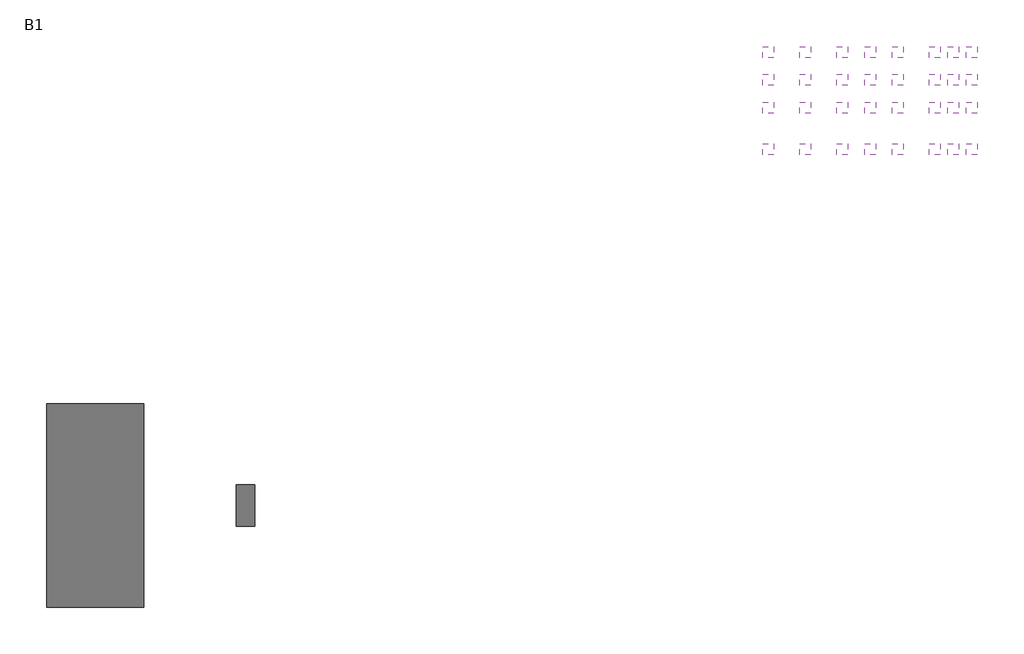
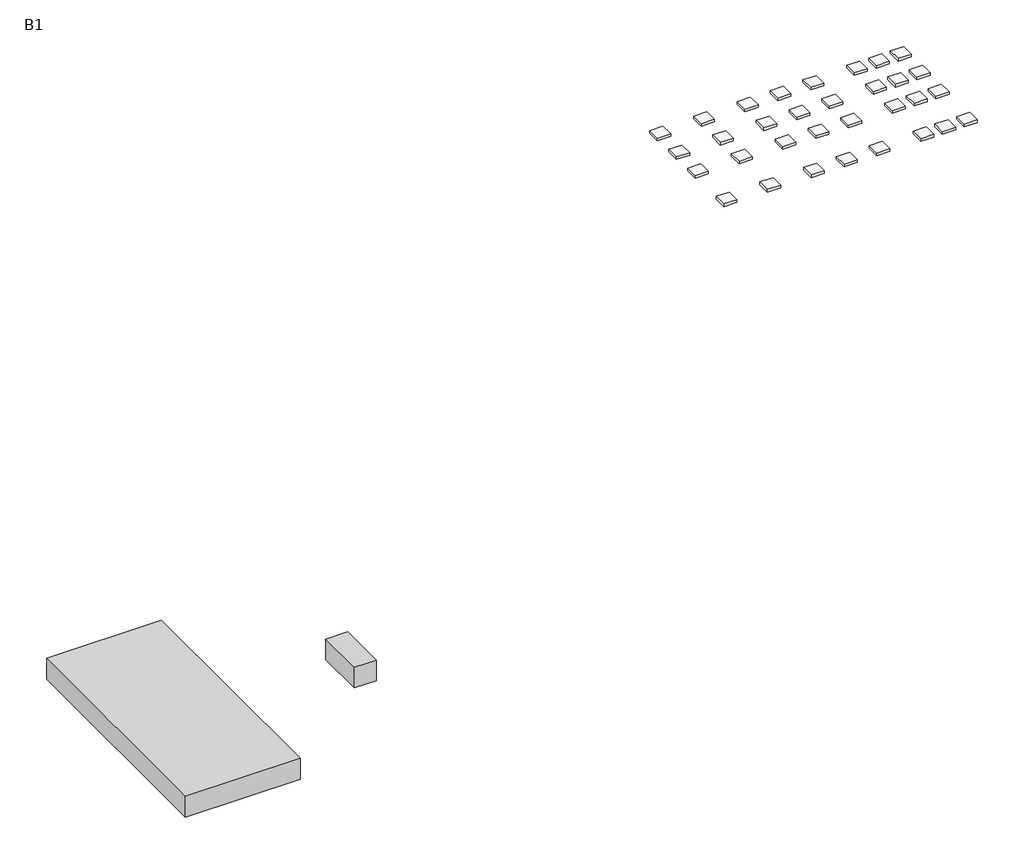
# One storey: 32 slabs, 2 proxies.
"""IFC4 building model written with IfcOpenShell, lengths in millimetres."""

import ifcopenshell
import ifcopenshell.guid

model = None  # the IFC model being written
_history = None  # IfcOwnerHistory: only IFC2X3 demands one
_inside = {}  # id of a spatial element -> (the spatial element, [elements in it])
_under = {}  # id of a project, library or spatial element -> (it, [spatial elements below it])
_declared = {}  # id of a project -> (the project, [libraries it declares])
_typed = {}  # id of a type object -> (the type object, [elements of that type])
_made_of = {}  # id of a material, layer set ... -> (it, [elements and type objects made of it])


def new_model(schema):
    """Start an empty IFC model of exactly this schema.

    Asked for "IFC4X3", IfcOpenShell would pick the latest addendum, in which some entities
    have other attributes; the version numbers below select the first issue.
    IFC2X3 requires an IfcOwnerHistory on every rooted entity: one is made here for all.
    """
    global model, _history
    if schema == "IFC4X3":
        model = ifcopenshell.file(schema_version=(4, 3, 0, 0))
    else:
        model = ifcopenshell.file(schema=schema)
    _inside.clear()
    _under.clear()
    _declared.clear()
    _typed.clear()
    _made_of.clear()
    _history = None
    if model.schema == "IFC2X3":
        org = make("IfcOrganization", Name="unknown")
        user = make(
            "IfcPersonAndOrganization",
            ThePerson=make("IfcPerson", FamilyName="unknown"),
            TheOrganization=org,
        )
        app = make(
            "IfcApplication",
            ApplicationDeveloper=org,
            Version="unknown",
            ApplicationFullName="unknown",
            ApplicationIdentifier="unknown",
        )
        _history = make(
            "IfcOwnerHistory",
            OwningUser=user,
            OwningApplication=app,
            ChangeAction="ADDED",
            CreationDate=0,
        )
    return model


def make(cls, **values):
    """One entity of the class cls with the attributes given. An attribute that is None is left unset."""
    return model.create_entity(
        cls, **{name: value for name, value in values.items() if value is not None}
    )


def rooted(cls, **values):
    """An entity with a GlobalId (a new one), such as an element, a storey or a relation."""
    return make(cls, GlobalId=ifcopenshell.guid.new(), OwnerHistory=_history, **values)


def si_unit(unit_type, name, prefix=None):
    """IfcSIUnit, for example si_unit("LENGTHUNIT", "METRE", prefix="MILLI")."""
    return make("IfcSIUnit", UnitType=unit_type, Prefix=prefix, Name=name)


def assignment(units):
    """IfcUnitAssignment: the units of a project."""
    return None if units is None else make("IfcUnitAssignment", Units=units)


def point(xyz):
    """IfcCartesianPoint."""
    return None if xyz is None else make("IfcCartesianPoint", Coordinates=xyz)


def direction(xyz):
    """IfcDirection."""
    return None if xyz is None else make("IfcDirection", DirectionRatios=xyz)


def frame(location, z_axis=None, x_axis=None):
    """IfcAxis2Placement3D, a coordinate frame: its origin and axes. An axis left out is left unset."""
    return make(
        "IfcAxis2Placement3D",
        Location=point(location),
        Axis=direction(z_axis),
        RefDirection=direction(x_axis),
    )


def origin():
    """The frame at (0, 0, 0) with its axes left unset."""
    return frame((0.0, 0.0, 0.0))


def origin_with_axes():
    """The frame at (0, 0, 0) with the z axis (0, 0, 1) and the x axis (1, 0, 0) written out."""
    return frame((0.0, 0.0, 0.0), z_axis=(0.0, 0.0, 1.0), x_axis=(1.0, 0.0, 0.0))


def place(relative_to, where):
    """IfcLocalPlacement: puts the frame where relative to a parent placement (None: the world)."""
    return make(
        "IfcLocalPlacement", PlacementRelTo=relative_to, RelativePlacement=where
    )


def context(
    kind, dimensions, precision=None, world=None, true_north=None, identifier=None
):
    """IfcGeometricRepresentationContext, for example the 3D "Model" context."""
    return make(
        "IfcGeometricRepresentationContext",
        ContextIdentifier=identifier,
        ContextType=kind,
        CoordinateSpaceDimension=dimensions,
        Precision=precision,
        WorldCoordinateSystem=world,
        TrueNorth=true_north,
    )


def project(units=None, contexts=None):
    """IfcProject with its units and contexts."""
    return rooted(
        "IfcProject",
        Name="project",
        RepresentationContexts=contexts,
        UnitsInContext=assignment(units),
    )


def spatial(cls, under=None, at=None, **own):
    """A site, building, storey or space (cls), placed at a placement, below another one or the project."""
    s = rooted(cls, ObjectPlacement=at, **own)
    if under is not None:
        _under.setdefault(under.id(), (under, []))[1].append(s)
    return s


def polyline(points):
    """IfcPolyline through the points."""
    return make("IfcPolyline", Points=[point(p) for p in points])


def outline(outer, holes=None, kind="AREA"):
    """IfcArbitraryClosedProfileDef: a profile drawn as a closed curve; with holes, ...WithVoids."""
    if holes is None:
        return make("IfcArbitraryClosedProfileDef", ProfileType=kind, OuterCurve=outer)
    return make(
        "IfcArbitraryProfileDefWithVoids",
        ProfileType=kind,
        OuterCurve=outer,
        InnerCurves=holes,
    )


def extrude(swept, where, along, depth):
    """IfcExtrudedAreaSolid: the profile swept, set in the frame where, extruded along a direction by depth."""
    return make(
        "IfcExtrudedAreaSolid",
        SweptArea=swept,
        Position=where,
        ExtrudedDirection=direction(along),
        Depth=depth,
    )


def shape(context_of_items, identifier, shape_type, items):
    """IfcShapeRepresentation: the items that make up one representation, for example the "Body"."""
    return make(
        "IfcShapeRepresentation",
        ContextOfItems=context_of_items,
        RepresentationIdentifier=identifier,
        RepresentationType=shape_type,
        Items=items,
    )


def source(mapping_origin, context_of_items, identifier, shape_type, items):
    """IfcRepresentationMap: a shape defined once, which mapped items show again and again."""
    return make(
        "IfcRepresentationMap",
        MappingOrigin=mapping_origin,
        MappedRepresentation=shape(context_of_items, identifier, shape_type, items),
    )


def transform(
    local_origin,
    x_axis=None,
    y_axis=None,
    z_axis=None,
    scale=None,
    scale2=None,
    scale3=None,
    uniform=True,
):
    """IfcCartesianTransformationOperator3D, or its non-uniform kind. x_axis, y_axis, z_axis: its Axis1, 2, 3."""
    if uniform:
        return make(
            "IfcCartesianTransformationOperator3D",
            Axis1=direction(x_axis),
            Axis2=direction(y_axis),
            LocalOrigin=point(local_origin),
            Scale=scale,
            Axis3=direction(z_axis),
        )
    return make(
        "IfcCartesianTransformationOperator3DnonUniform",
        Axis1=direction(x_axis),
        Axis2=direction(y_axis),
        LocalOrigin=point(local_origin),
        Scale=scale,
        Axis3=direction(z_axis),
        Scale2=scale2,
        Scale3=scale3,
    )


def mapped(mapping_source, mapping_target):
    """IfcMappedItem: shows the shape of a source again, moved by a transform."""
    return make(
        "IfcMappedItem", MappingSource=mapping_source, MappingTarget=mapping_target
    )


def made_of(thing, what):
    """Note that an element or type object is made of a material, layer set ...; save() writes the relation."""
    if what is not None:
        _made_of.setdefault(what.id(), (what, []))[1].append(thing)
    return thing


def element(
    cls,
    number,
    at=None,
    inside=None,
    cuts=None,
    type_object=None,
    material=None,
    context=None,
    identifier="Body",
    shape_type=None,
    held_by="IfcProductDefinitionShape",
    body=None,
    shapes=None,
    **own,
):
    """One element of the class cls, such as IfcWall. Its Tag is "e" and its number.

    at: its placement. inside: the storey or other place that contains it. cuts: it is an
    opening in that element (IfcRelVoidsElement). A single representation is given by context,
    identifier, shape_type and body (its items); several are given by shapes. held_by: the class
    of the entity that holds the representations. save() writes the other relations.
    """
    e = rooted(cls, Tag="e%d" % number, ObjectPlacement=at, **own)
    if body is not None:
        shapes = [shape(context, identifier, shape_type, body)]
    if shapes is not None:
        e.Representation = make(held_by, Representations=shapes)
    if inside is not None:
        _inside.setdefault(inside.id(), (inside, []))[1].append(e)
    if cuts is not None:
        rooted(
            "IfcRelVoidsElement", RelatingBuildingElement=cuts, RelatedOpeningElement=e
        )
    if type_object is not None:
        _typed.setdefault(type_object.id(), (type_object, []))[1].append(e)
    return made_of(e, material)


def aggregate(whole, parts):
    """IfcRelAggregates: a whole, such as a stair, and the parts it consists of."""
    return rooted("IfcRelAggregates", RelatingObject=whole, RelatedObjects=parts)


def save(model, path):
    """Write the relations noted so far, then the file.

    IfcRelAggregates (storeys below a building ...), IfcRelContainedInSpatialStructure (elements
    in a storey), IfcRelDefinesByType, IfcRelAssociatesMaterial and IfcRelDeclares: one each for
    every whole, place, type object, material and project.
    """
    for whole, parts in _under.values():
        aggregate(whole, parts)
    for where, things in _inside.values():
        rooted(
            "IfcRelContainedInSpatialStructure",
            RelatedElements=things,
            RelatingStructure=where,
        )
    for kind, things in _typed.values():
        rooted("IfcRelDefinesByType", RelatedObjects=things, RelatingType=kind)
    for what, things in _made_of.values():
        rooted("IfcRelAssociatesMaterial", RelatedObjects=things, RelatingMaterial=what)
    for by, libraries in _declared.values():
        rooted("IfcRelDeclares", RelatingContext=by, RelatedDefinitions=libraries)
    model.write(path)


def generic_models_a454a2aa(model_context):
    return source(origin(), model_context, "Body", "SweptSolid", [
        extrude(outline(polyline([(10500.0, 22000.0), (10500.0, -22000.0), (-10500.0, -22000.0), (-10500.0, 22000.0), (10500.0, 22000.0)])), origin_with_axes(), (0.0, 0.0, 1.0), 4000.0),
    ])


def generic_models_73802227(model_context):
    return source(origin(), model_context, "Body", "SweptSolid", [
        extrude(outline(polyline([(2000.0, 4500.0), (2000.0, -4500.0), (-2000.0, -4500.0), (-2000.0, 4500.0), (2000.0, 4500.0)])), origin_with_axes(), (0.0, 0.0, 1.0), 4000.0),
    ])


def ft112_footing_rectangular_ft112_2400x2400x500_5fe39465(model_context):
    return source(origin(), model_context, "Body", "SweptSolid", [
        extrude(outline(polyline([(1200.0, 1200.0), (1200.0, -1200.0), (-1200.0, -1200.0), (-1200.0, 1200.0), (1200.0, 1200.0)])), frame((0.0, 0.0, -500.0), z_axis=(0.0, 0.0, 1.0), x_axis=(1.0, 0.0, 0.0)), (0.0, 0.0, 1.0), 500.0),
    ])


model = new_model("IFC4")

# Units and contexts
model_context = context("Model", 3, world=origin())
ifc_project = project(units=[si_unit("LENGTHUNIT", "METRE", prefix="MILLI")], contexts=[model_context])

# Site, building, storey
site = spatial("IfcSite", under=ifc_project)
building = spatial("IfcBuilding", under=site)
storey = spatial("IfcBuildingStorey", under=building, Name="B1", Elevation=-5000.0)

# Proxies
placement = place(None, origin())
generic_models_shape = generic_models_a454a2aa(model_context)
element("IfcBuildingElementProxy", 1, Name="Space Planning Box_hec : Space Planning Box_hec", ObjectType="Space Planning Box_hec : Space Planning Box_hec", at=placement, inside=storey, context=model_context, shape_type="MappedRepresentation", body=[
    mapped(generic_models_shape, transform((10500.0, 54000.0, -5000.0), x_axis=(1.0, 0.0, 0.0), y_axis=(0.0, 1.0, 0.0), z_axis=(0.0, 0.0, 1.0))),
])
generic_models_2_shape = generic_models_73802227(model_context)
element("IfcBuildingElementProxy", 2, Name="Space Planning Box_hec : Space Planning Box_hec", ObjectType="Space Planning Box_hec : Space Planning Box_hec", at=placement, inside=storey, context=model_context, shape_type="MappedRepresentation", body=[
    mapped(generic_models_2_shape, transform((43000.0, 54000.0, -5000.0), x_axis=(1.0, 0.0, 0.0), y_axis=(0.0, 1.0, 0.0), z_axis=(0.0, 0.0, 1.0))),
])

# Slabs
ft112_footing_rectangular_ft112_2400x2400x500_shape = ft112_footing_rectangular_ft112_2400x2400x500_5fe39465(model_context)
element("IfcSlab", 3, ObjectType="FT112-Footing-Rectangular : FT112_2400x2400x500", at=placement, inside=storey, context=model_context, shape_type="MappedRepresentation", body=[
    mapped(ft112_footing_rectangular_ft112_2400x2400x500_shape, transform((156114.1020501, 152015.7581198, 0.0), x_axis=(1.0, 0.0, 0.0), y_axis=(0.0, 1.0, 0.0), z_axis=(0.0, 0.0, 1.0))),
])
element("IfcSlab", 4, ObjectType="FT112-Footing-Rectangular : FT112_2400x2400x500", at=placement, inside=storey, context=model_context, shape_type="MappedRepresentation", body=[
    mapped(ft112_footing_rectangular_ft112_2400x2400x500_shape, transform((156114.1020501, 146015.7581198, 0.0), x_axis=(1.0, 0.0, 0.0), y_axis=(0.0, 1.0, 0.0), z_axis=(0.0, 0.0, 1.0))),
])
element("IfcSlab", 5, ObjectType="FT112-Footing-Rectangular : FT112_2400x2400x500", at=placement, inside=storey, context=model_context, shape_type="MappedRepresentation", body=[
    mapped(ft112_footing_rectangular_ft112_2400x2400x500_shape, transform((156114.1020501, 140015.7581198, 0.0), x_axis=(1.0, 0.0, 0.0), y_axis=(0.0, 1.0, 0.0), z_axis=(0.0, 0.0, 1.0))),
])
element("IfcSlab", 6, ObjectType="FT112-Footing-Rectangular : FT112_2400x2400x500", at=placement, inside=storey, context=model_context, shape_type="MappedRepresentation", body=[
    mapped(ft112_footing_rectangular_ft112_2400x2400x500_shape, transform((156114.1020501, 131015.7581198, 0.0), x_axis=(1.0, 0.0, 0.0), y_axis=(0.0, 1.0, 0.0), z_axis=(0.0, 0.0, 1.0))),
])
element("IfcSlab", 7, ObjectType="FT112-Footing-Rectangular : FT112_2400x2400x500", at=placement, inside=storey, context=model_context, shape_type="MappedRepresentation", body=[
    mapped(ft112_footing_rectangular_ft112_2400x2400x500_shape, transform((164114.1020501, 152015.7581198, 0.0), x_axis=(1.0, 0.0, 0.0), y_axis=(0.0, 1.0, 0.0), z_axis=(0.0, 0.0, 1.0))),
])
element("IfcSlab", 8, ObjectType="FT112-Footing-Rectangular : FT112_2400x2400x500", at=placement, inside=storey, context=model_context, shape_type="MappedRepresentation", body=[
    mapped(ft112_footing_rectangular_ft112_2400x2400x500_shape, transform((164114.1020501, 146015.7581198, 0.0), x_axis=(1.0, 0.0, 0.0), y_axis=(0.0, 1.0, 0.0), z_axis=(0.0, 0.0, 1.0))),
])
element("IfcSlab", 9, ObjectType="FT112-Footing-Rectangular : FT112_2400x2400x500", at=placement, inside=storey, context=model_context, shape_type="MappedRepresentation", body=[
    mapped(ft112_footing_rectangular_ft112_2400x2400x500_shape, transform((164114.1020501, 140015.7581198, 0.0), x_axis=(1.0, 0.0, 0.0), y_axis=(0.0, 1.0, 0.0), z_axis=(0.0, 0.0, 1.0))),
])
element("IfcSlab", 10, ObjectType="FT112-Footing-Rectangular : FT112_2400x2400x500", at=placement, inside=storey, context=model_context, shape_type="MappedRepresentation", body=[
    mapped(ft112_footing_rectangular_ft112_2400x2400x500_shape, transform((164114.1020501, 131015.7581198, 0.0), x_axis=(1.0, 0.0, 0.0), y_axis=(0.0, 1.0, 0.0), z_axis=(0.0, 0.0, 1.0))),
])
element("IfcSlab", 11, ObjectType="FT112-Footing-Rectangular : FT112_2400x2400x500", at=placement, inside=storey, context=model_context, shape_type="MappedRepresentation", body=[
    mapped(ft112_footing_rectangular_ft112_2400x2400x500_shape, transform((172114.1020501, 152015.7581198, 0.0), x_axis=(1.0, 0.0, 0.0), y_axis=(0.0, 1.0, 0.0), z_axis=(0.0, 0.0, 1.0))),
])
element("IfcSlab", 12, ObjectType="FT112-Footing-Rectangular : FT112_2400x2400x500", at=placement, inside=storey, context=model_context, shape_type="MappedRepresentation", body=[
    mapped(ft112_footing_rectangular_ft112_2400x2400x500_shape, transform((172114.1020501, 146015.7581198, 0.0), x_axis=(1.0, 0.0, 0.0), y_axis=(0.0, 1.0, 0.0), z_axis=(0.0, 0.0, 1.0))),
])
element("IfcSlab", 13, ObjectType="FT112-Footing-Rectangular : FT112_2400x2400x500", at=placement, inside=storey, context=model_context, shape_type="MappedRepresentation", body=[
    mapped(ft112_footing_rectangular_ft112_2400x2400x500_shape, transform((172114.1020501, 140015.7581198, 0.0), x_axis=(1.0, 0.0, 0.0), y_axis=(0.0, 1.0, 0.0), z_axis=(0.0, 0.0, 1.0))),
])
element("IfcSlab", 14, ObjectType="FT112-Footing-Rectangular : FT112_2400x2400x500", at=placement, inside=storey, context=model_context, shape_type="MappedRepresentation", body=[
    mapped(ft112_footing_rectangular_ft112_2400x2400x500_shape, transform((172114.1020501, 131015.7581198, 0.0), x_axis=(1.0, 0.0, 0.0), y_axis=(0.0, 1.0, 0.0), z_axis=(0.0, 0.0, 1.0))),
])
element("IfcSlab", 15, ObjectType="FT112-Footing-Rectangular : FT112_2400x2400x500", at=placement, inside=storey, context=model_context, shape_type="MappedRepresentation", body=[
    mapped(ft112_footing_rectangular_ft112_2400x2400x500_shape, transform((178114.1020501, 152015.7581198, 0.0), x_axis=(1.0, 0.0, 0.0), y_axis=(0.0, 1.0, 0.0), z_axis=(0.0, 0.0, 1.0))),
])
element("IfcSlab", 16, ObjectType="FT112-Footing-Rectangular : FT112_2400x2400x500", at=placement, inside=storey, context=model_context, shape_type="MappedRepresentation", body=[
    mapped(ft112_footing_rectangular_ft112_2400x2400x500_shape, transform((178114.1020501, 146015.7581198, 0.0), x_axis=(1.0, 0.0, 0.0), y_axis=(0.0, 1.0, 0.0), z_axis=(0.0, 0.0, 1.0))),
])
element("IfcSlab", 17, ObjectType="FT112-Footing-Rectangular : FT112_2400x2400x500", at=placement, inside=storey, context=model_context, shape_type="MappedRepresentation", body=[
    mapped(ft112_footing_rectangular_ft112_2400x2400x500_shape, transform((178114.1020501, 140015.7581198, 0.0), x_axis=(1.0, 0.0, 0.0), y_axis=(0.0, 1.0, 0.0), z_axis=(0.0, 0.0, 1.0))),
])
element("IfcSlab", 18, ObjectType="FT112-Footing-Rectangular : FT112_2400x2400x500", at=placement, inside=storey, context=model_context, shape_type="MappedRepresentation", body=[
    mapped(ft112_footing_rectangular_ft112_2400x2400x500_shape, transform((178114.1020501, 131015.7581198, 0.0), x_axis=(1.0, 0.0, 0.0), y_axis=(0.0, 1.0, 0.0), z_axis=(0.0, 0.0, 1.0))),
])
element("IfcSlab", 19, ObjectType="FT112-Footing-Rectangular : FT112_2400x2400x500", at=placement, inside=storey, context=model_context, shape_type="MappedRepresentation", body=[
    mapped(ft112_footing_rectangular_ft112_2400x2400x500_shape, transform((184114.1020501, 152015.7581198, 0.0), x_axis=(1.0, 0.0, 0.0), y_axis=(0.0, 1.0, 0.0), z_axis=(0.0, 0.0, 1.0))),
])
element("IfcSlab", 20, ObjectType="FT112-Footing-Rectangular : FT112_2400x2400x500", at=placement, inside=storey, context=model_context, shape_type="MappedRepresentation", body=[
    mapped(ft112_footing_rectangular_ft112_2400x2400x500_shape, transform((184114.1020501, 146015.7581198, 0.0), x_axis=(1.0, 0.0, 0.0), y_axis=(0.0, 1.0, 0.0), z_axis=(0.0, 0.0, 1.0))),
])
element("IfcSlab", 21, ObjectType="FT112-Footing-Rectangular : FT112_2400x2400x500", at=placement, inside=storey, context=model_context, shape_type="MappedRepresentation", body=[
    mapped(ft112_footing_rectangular_ft112_2400x2400x500_shape, transform((184114.1020501, 140015.7581198, 0.0), x_axis=(1.0, 0.0, 0.0), y_axis=(0.0, 1.0, 0.0), z_axis=(0.0, 0.0, 1.0))),
])
element("IfcSlab", 22, ObjectType="FT112-Footing-Rectangular : FT112_2400x2400x500", at=placement, inside=storey, context=model_context, shape_type="MappedRepresentation", body=[
    mapped(ft112_footing_rectangular_ft112_2400x2400x500_shape, transform((184114.1020501, 131015.7581198, 0.0), x_axis=(1.0, 0.0, 0.0), y_axis=(0.0, 1.0, 0.0), z_axis=(0.0, 0.0, 1.0))),
])
element("IfcSlab", 23, ObjectType="FT112-Footing-Rectangular : FT112_2400x2400x500", at=placement, inside=storey, context=model_context, shape_type="MappedRepresentation", body=[
    mapped(ft112_footing_rectangular_ft112_2400x2400x500_shape, transform((192114.1020501, 152015.7581198, 0.0), x_axis=(1.0, 0.0, 0.0), y_axis=(0.0, 1.0, 0.0), z_axis=(0.0, 0.0, 1.0))),
])
element("IfcSlab", 24, ObjectType="FT112-Footing-Rectangular : FT112_2400x2400x500", at=placement, inside=storey, context=model_context, shape_type="MappedRepresentation", body=[
    mapped(ft112_footing_rectangular_ft112_2400x2400x500_shape, transform((192114.1020501, 146015.7581198, 0.0), x_axis=(1.0, 0.0, 0.0), y_axis=(0.0, 1.0, 0.0), z_axis=(0.0, 0.0, 1.0))),
])
element("IfcSlab", 25, ObjectType="FT112-Footing-Rectangular : FT112_2400x2400x500", at=placement, inside=storey, context=model_context, shape_type="MappedRepresentation", body=[
    mapped(ft112_footing_rectangular_ft112_2400x2400x500_shape, transform((192114.1020501, 140015.7581198, 0.0), x_axis=(1.0, 0.0, 0.0), y_axis=(0.0, 1.0, 0.0), z_axis=(0.0, 0.0, 1.0))),
])
element("IfcSlab", 26, ObjectType="FT112-Footing-Rectangular : FT112_2400x2400x500", at=placement, inside=storey, context=model_context, shape_type="MappedRepresentation", body=[
    mapped(ft112_footing_rectangular_ft112_2400x2400x500_shape, transform((192114.1020501, 131015.7581198, 0.0), x_axis=(1.0, 0.0, 0.0), y_axis=(0.0, 1.0, 0.0), z_axis=(0.0, 0.0, 1.0))),
])
element("IfcSlab", 27, ObjectType="FT112-Footing-Rectangular : FT112_2400x2400x500", at=placement, inside=storey, context=model_context, shape_type="MappedRepresentation", body=[
    mapped(ft112_footing_rectangular_ft112_2400x2400x500_shape, transform((196114.1020501, 152015.7581198, 0.0), x_axis=(1.0, 0.0, 0.0), y_axis=(0.0, 1.0, 0.0), z_axis=(0.0, 0.0, 1.0))),
])
element("IfcSlab", 28, ObjectType="FT112-Footing-Rectangular : FT112_2400x2400x500", at=placement, inside=storey, context=model_context, shape_type="MappedRepresentation", body=[
    mapped(ft112_footing_rectangular_ft112_2400x2400x500_shape, transform((196114.1020501, 146015.7581198, 0.0), x_axis=(1.0, 0.0, 0.0), y_axis=(0.0, 1.0, 0.0), z_axis=(0.0, 0.0, 1.0))),
])
element("IfcSlab", 29, ObjectType="FT112-Footing-Rectangular : FT112_2400x2400x500", at=placement, inside=storey, context=model_context, shape_type="MappedRepresentation", body=[
    mapped(ft112_footing_rectangular_ft112_2400x2400x500_shape, transform((196114.1020501, 140015.7581198, 0.0), x_axis=(1.0, 0.0, 0.0), y_axis=(0.0, 1.0, 0.0), z_axis=(0.0, 0.0, 1.0))),
])
element("IfcSlab", 30, ObjectType="FT112-Footing-Rectangular : FT112_2400x2400x500", at=placement, inside=storey, context=model_context, shape_type="MappedRepresentation", body=[
    mapped(ft112_footing_rectangular_ft112_2400x2400x500_shape, transform((196114.1020501, 131015.7581198, 0.0), x_axis=(1.0, 0.0, 0.0), y_axis=(0.0, 1.0, 0.0), z_axis=(0.0, 0.0, 1.0))),
])
element("IfcSlab", 31, ObjectType="FT112-Footing-Rectangular : FT112_2400x2400x500", at=placement, inside=storey, context=model_context, shape_type="MappedRepresentation", body=[
    mapped(ft112_footing_rectangular_ft112_2400x2400x500_shape, transform((200114.1020501, 152015.7581198, 0.0), x_axis=(1.0, 0.0, 0.0), y_axis=(0.0, 1.0, 0.0), z_axis=(0.0, 0.0, 1.0))),
])
element("IfcSlab", 32, ObjectType="FT112-Footing-Rectangular : FT112_2400x2400x500", at=placement, inside=storey, context=model_context, shape_type="MappedRepresentation", body=[
    mapped(ft112_footing_rectangular_ft112_2400x2400x500_shape, transform((200114.1020501, 146015.7581198, 0.0), x_axis=(1.0, 0.0, 0.0), y_axis=(0.0, 1.0, 0.0), z_axis=(0.0, 0.0, 1.0))),
])
element("IfcSlab", 33, ObjectType="FT112-Footing-Rectangular : FT112_2400x2400x500", at=placement, inside=storey, context=model_context, shape_type="MappedRepresentation", body=[
    mapped(ft112_footing_rectangular_ft112_2400x2400x500_shape, transform((200114.1020501, 140015.7581198, 0.0), x_axis=(1.0, 0.0, 0.0), y_axis=(0.0, 1.0, 0.0), z_axis=(0.0, 0.0, 1.0))),
])
element("IfcSlab", 34, ObjectType="FT112-Footing-Rectangular : FT112_2400x2400x500", at=placement, inside=storey, context=model_context, shape_type="MappedRepresentation", body=[
    mapped(ft112_footing_rectangular_ft112_2400x2400x500_shape, transform((200114.1020501, 131015.7581198, 0.0), x_axis=(1.0, 0.0, 0.0), y_axis=(0.0, 1.0, 0.0), z_axis=(0.0, 0.0, 1.0))),
])

save(model, "model.ifc")

# Revit data of these elements
# Project information
#   Project Issue Date = "Issue Date"
#   Project Status = "Project Status"
#   Client Name = "Owner"
#   Project Address = "Enter address here"
#   Project Name = "Project Name"
#   Project Number = "Project Number"
# Grids (mm)
#   "A": line (156114.102, 123537.292) -> (156114.102, 157930.913)
#   "B": line (164114.102, 123537.292) -> (164114.102, 157930.913)
#   "C": line (172114.102, 123537.292) -> (172114.102, 157930.913)
#   "D": line (178114.102, 123537.292) -> (178114.102, 157930.913)
#   "E": line (184114.102, 123537.292) -> (184114.102, 157930.913)
#   "F": line (192114.102, 123537.292) -> (192114.102, 157930.913)
#   "G": line (196114.102, 123537.292) -> (196114.102, 157930.913)
#   "8": line (145724.678, 152015.758) -> (209069.776, 152015.758)
#   "3": line (145724.678, 146015.758) -> (209069.776, 146015.758)
#   "2": line (145724.678, 140015.758) -> (209069.776, 140015.758)
#   "1": line (145724.678, 131015.758) -> (209069.776, 131015.758)
#   "H": line (200114.102, 123537.292) -> (200114.102, 157930.913)
# Type "Space Planning Box_hec : Space Planning Box_hec"
#   Type Comments = "..."
#   Room Name [instance default] = "?"
#   Interior Finish [instance default] = ""
#   Exterior Finish [instance default] = ""
#   Department [instance default] = ""
#   Assembly Code = "..."
#   Width [instance default] = 1524 mm
#   Program Area [instance default] = 0 m²
#   Length [instance default] = 1524 mm
#   Height [instance default] = 1524 mm
#   Area [instance default] = 2.32258 m²
#   Fill Color [instance default] = Cyan
#   Default Elevation = 0
# Type "FT112-Footing-Rectangular : FT112_2400x2400x500"
#   Description = "UG Shallow Foundation"
#   Width = 2400 mm
#   Length = 2400 mm
#   Foundation Thickness = 500 mm
#   hec_material3 [instance default] = none
#   hec_material2 [instance default] = A03AE056-00001_Bitumen/Bituminous/Asphalt Coating
#   hec_material1 [instance default] = A03AC035-00001_Form Work (3 times in use)_Flat
#   Structural Material [instance default] = A03AC032-00007_Structural Concrete_Type1_25MPa-30Mpa
#   Assembly Code = ""
# Element 1 (IfcBuildingElementProxy, "Space Planning Box_hec : Space Planning Box_hec")
#   Room Name = "Cable Room"
#   Interior Finish = "IF1"
#   Exterior Finish = "EF1"
#   Department = "EL"
#   Width = 21000 mm
#   Program Area = 924 m²
#   Length = 44000 mm
#   Height = 4000 mm
#   Area = 924 m²
#   Fill Color = Blue
#   Phase Created = New Construction
#   Materials on its faces: "Blue"
# Element 2 (IfcBuildingElementProxy, "Space Planning Box_hec : Space Planning Box_hec")
#   Room Name = "Stairway"
#   Interior Finish = "IF2"
#   Exterior Finish = "EF1"
#   Department = "EL"
#   Width = 4000 mm
#   Program Area = 36 m²
#   Length = 9000 mm
#   Height = 4000 mm
#   Area = 36 m²
#   Fill Color = Blue
#   Phase Created = New Construction
#   Materials on its faces: "Blue"
# Elements 3, 4, 5, 6, 7, 8, 9, 10, 11, 12, 13, 14, 15, 16, 17, 18, 19, 20, 21, 22, 23, 24, 25, 26, 27, 28, 29, 30, 31, 32, 33, 34 (IfcSlab, "FT112-Footing-Rectangular : FT112_2400x2400x500")
#   hec_material3 = none
#   hec_material2 = A03AE056-00001_Bitumen/Bituminous/Asphalt Coating
#   hec_material1 = A03AC035-00001_Form Work (3 times in use)_Flat
#   Structural Material = A03AC032-00007_Structural Concrete_Type1_25MPa-30Mpa
#   Phase Created = New Construction
#   Materials on its faces: "A03AC032-00007_Structural Concrete_Type1_25MPa-30Mpa"
# Materials
#   "Cyan": class "Generic", colour RGB 0 255 255, transparency 0.2, Cost = 0
#   "A03AE056-00001_Bitumen/Bituminous/Asphalt Coating": class "Generic", colour RGB 17 17 17, transparency 0, Description = "Damp-proofing", W00) Work Master Code = "A03AE056-00001", W01) Work Master_Lv1 = "Concrete Work", W02) Work Master_Lv2 = "Concrete Protective Coating (U/G)", W03) Work Master_Spec.1 = "Bitumen/Bituminous/Asphalt Coating", Cost = 0
#   "A03AC035-00001_Form Work (3 times in use)_Flat": class "Wood", colour RGB 149 120 74, transparency 0, Description = "Plywood", W00) Work Master Code = "A03AC035-00001", W01) Work Master_Lv1 = "Concrete Work", W02) Work Master_Lv2 = "Substructure Work", W03) Work Master_Spec.1 = "Form Work (3 times in use)", W04) Work Master_Spec.2 = "Flat Form", W05) Work Master_Spec.3 = "Dressed Lumber, Plywood or Steel Form(Wood Planks are not Allowed) incl. Chamfer", Cost = 0
#   "A03AC032-00007_Structural Concrete_Type1_25MPa-30Mpa": class "Concrete", colour RGB 176 176 176, transparency 0, Keynote = "09910.A1", Description = "Reinf. Conc.", W00) Work Master Code = "A03AC032-00007", W01) Work Master_Lv1 = "Concrete Work", W02) Work Master_Lv2 = "Substructure Work", W03) Work Master_Spec.1 = "Structural Concrete", W04) Work Master_Spec.2 = "Cement Type-1", W05) Work Master_Spec.3 = "25MPa < F'c (Cylinder Strength) ≤ 30MPa", Cost = 0
#   "Blue": class "Generic", colour RGB 0 0 255, transparency 0.2, Cost = 0
